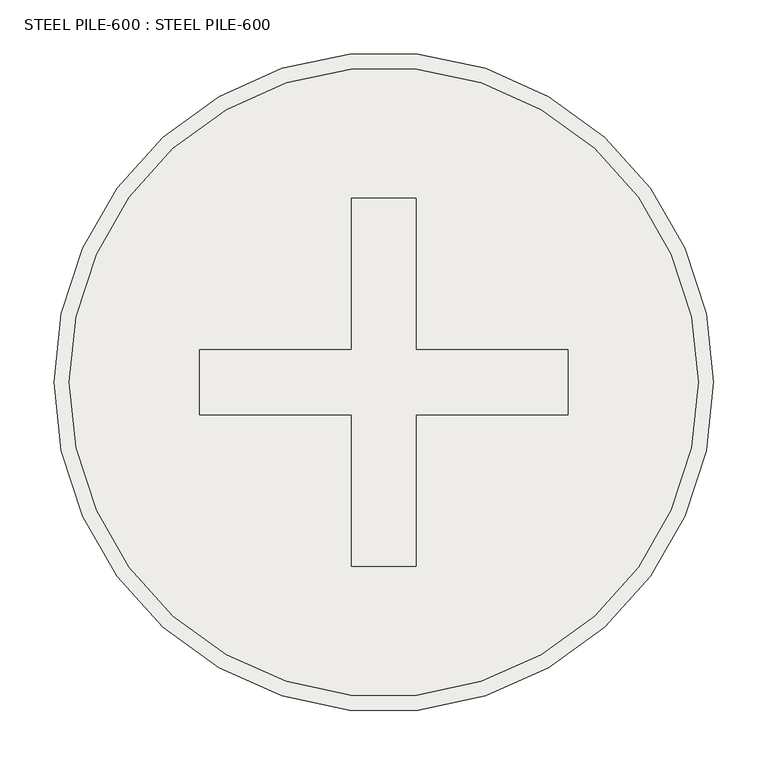
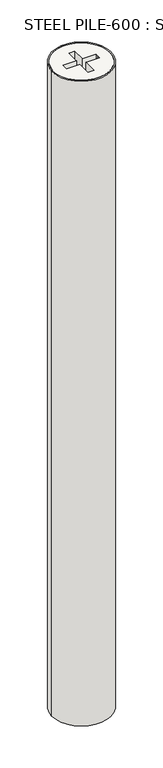
"""IFC4 building model written with IfcOpenShell, lengths in millimetres: slab geometry, STEEL PILE-600 : STEEL PILE-600."""

from ifc_helpers import new_model, si_unit, point, frame, frame_2d, origin, place, context, project, spatial, circle_curve, trimmed, segment, composite_curve, outline, extrude, source, transform, mapped, element, save
from ifc_brep_helpers import plane_surface, cylinder_surface, advanced_brep


def steel_pile_600_steel_pile_600_e2eeaf4c(model_context):
    return source(origin(), model_context, "Body", "SolidModel", [
        advanced_brep(
        [(-290.5, 19499.5208589, 150.0), (290.5, 19499.5208589, 150.0), (-30.0, 19469.5208589, 150.0), (-170.0, 19469.5208589, 150.0), (-170.0, 19499.5208589, 150.0), (-170.0, 19529.5208589, 150.0), (-30.0, 19529.5208589, 150.0), (-30.0, 19669.5208589, 150.0), (30.0, 19669.5208589, 150.0), (30.0, 19529.5208589, 150.0), (170.0, 19529.5208589, 150.0), (170.0, 19499.5208589, 150.0), (170.0, 19469.5208589, 150.0), (30.0, 19469.5208589, 150.0), (30.0, 19329.5208589, 150.0), (-30.0, 19329.5208589, 150.0), (-290.5, 19499.5208589, -1850.0), (290.5, 19499.5208589, -1850.0), (-170.0, 19469.5208589, -160.0), (-30.0, 19469.5208589, -160.0), (-30.0, 19329.5208589, -160.0), (30.0, 19329.5208589, -160.0), (30.0, 19469.5208589, -160.0), (170.0, 19469.5208589, -160.0), (170.0, 19499.5208589, -160.0), (170.0, 19529.5208589, -160.0), (30.0, 19529.5208589, -160.0), (30.0, 19669.5208589, -160.0), (-30.0, 19669.5208589, -160.0), (-30.0, 19529.5208589, -160.0), (-170.0, 19529.5208589, -160.0), (-170.0, 19499.5208589, -160.0)],
        [
            (0, 1, circle_curve(frame((0.0, 19499.5208589, 150.0), z_axis=(0.0, 0.0, 1.0), x_axis=(1.0, 0.0, 0.0)), 290.5)),
            (1, 0, circle_curve(frame((0.0, 19499.5208589, 150.0), z_axis=(0.0, 0.0, 1.0), x_axis=(1.0, 0.0, 0.0)), 290.5)),
            (2, 3),
            (3, 4),
            (4, 5),
            (5, 6),
            (6, 7),
            (7, 8),
            (8, 9),
            (9, 10),
            (10, 11),
            (11, 12),
            (12, 13),
            (13, 14),
            (14, 15),
            (15, 2),
            (16, 17, circle_curve(frame((0.0, 19499.5208589, -1850.0), z_axis=(0.0, 0.0, -1.0), x_axis=(1.0, 0.0, 0.0)), 290.5)),
            (17, 16, circle_curve(frame((0.0, 19499.5208589, -1850.0), z_axis=(0.0, 0.0, -1.0), x_axis=(1.0, 0.0, 0.0)), 290.5)),
            (0, 16),
            (17, 1),
            (18, 19),
            (19, 20),
            (20, 21),
            (21, 22),
            (22, 23),
            (23, 24),
            (24, 25),
            (25, 26),
            (26, 27),
            (27, 28),
            (28, 29),
            (29, 30),
            (30, 31),
            (31, 18),
            (18, 3),
            (2, 19),
            (15, 20),
            (14, 21),
            (13, 22),
            (12, 23),
            (11, 24),
            (10, 25),
            (9, 26),
            (8, 27),
            (7, 28),
            (6, 29),
            (5, 30),
            (4, 31),
        ],
        [
            plane_surface(frame((290.5, 19499.5208589, 150.0), z_axis=(0.0, 0.0, 1.0), x_axis=(0.0, 1.0, 0.0))),
            plane_surface(frame((290.5, 19499.5208589, -1850.0), z_axis=(0.0, 0.0, -1.0), x_axis=(0.0, -1.0, 0.0))),
            cylinder_surface(frame((0.0, 19499.5208589, -1850.0), z_axis=(0.0, 0.0, 1.0), x_axis=(1.0, 0.0, 0.0)), 290.5),
            plane_surface(frame((-170.0, 19469.5208589, -160.0), z_axis=(0.0, 0.0, 1.0), x_axis=(-1.0, 0.0, 0.0))),
            plane_surface(frame((-170.0, 19469.5208589, 160.0), z_axis=(0.0, 1.0, 0.0), x_axis=(0.0, 0.0, -1.0))),
            plane_surface(frame((-30.0, 19469.5208589, 160.0), z_axis=(1.0, 0.0, 0.0), x_axis=(0.0, 0.0, -1.0))),
            plane_surface(frame((-30.0, 19329.5208589, 160.0), z_axis=(0.0, 1.0, 0.0), x_axis=(0.0, 0.0, -1.0))),
            plane_surface(frame((30.0, 19329.5208589, 160.0), z_axis=(-1.0, 0.0, 0.0), x_axis=(0.0, 0.0, -1.0))),
            plane_surface(frame((30.0, 19469.5208589, 160.0), z_axis=(0.0, 1.0, 0.0), x_axis=(0.0, 0.0, -1.0))),
            plane_surface(frame((170.0, 19469.5208589, 160.0), z_axis=(-1.0, 0.0, 0.0), x_axis=(0.0, 0.0, -1.0))),
            plane_surface(frame((170.0, 19499.5208589, 160.0), z_axis=(-1.0, 0.0, 0.0), x_axis=(0.0, 0.0, -1.0))),
            plane_surface(frame((170.0, 19529.5208589, 160.0), z_axis=(0.0, -1.0, 0.0), x_axis=(0.0, 0.0, -1.0))),
            plane_surface(frame((30.0, 19529.5208589, 160.0), z_axis=(-1.0, 0.0, 0.0), x_axis=(0.0, 0.0, -1.0))),
            plane_surface(frame((30.0, 19669.5208589, 160.0), z_axis=(0.0, -1.0, 0.0), x_axis=(0.0, 0.0, -1.0))),
            plane_surface(frame((-30.0, 19669.5208589, 160.0), z_axis=(1.0, 0.0, 0.0), x_axis=(0.0, 0.0, -1.0))),
            plane_surface(frame((-30.0, 19529.5208589, 160.0), z_axis=(0.0, -1.0, 0.0), x_axis=(0.0, 0.0, -1.0))),
            plane_surface(frame((-170.0, 19529.5208589, 160.0), z_axis=(1.0, 0.0, 0.0), x_axis=(0.0, 0.0, -1.0))),
            plane_surface(frame((-170.0, 19499.5208589, 160.0), z_axis=(1.0, 0.0, 0.0), x_axis=(0.0, 0.0, -1.0))),
        ],
        [
            (0, [[1, 2], [3, 4, 5, 6, 7, 8, 9, 10, 11, 12, 13, 14, 15, 16]]),
            (1, [[17, 18]]),
            (2, [[-1, 19, -18, 20]]),
            (2, [[-2, -20, -17, -19]]),
            (3, [[21, 22, 23, 24, 25, 26, 27, 28, 29, 30, 31, 32, 33, 34]]),
            (4, [[-21, 35, -3, 36]]),
            (5, [[-22, -36, -16, 37]]),
            (6, [[-23, -37, -15, 38]]),
            (7, [[-24, -38, -14, 39]]),
            (8, [[-25, -39, -13, 40]]),
            (9, [[-26, -40, -12, 41]]),
            (10, [[-27, -41, -11, 42]]),
            (11, [[-28, -42, -10, 43]]),
            (12, [[-29, -43, -9, 44]]),
            (13, [[-30, -44, -8, 45]]),
            (14, [[-31, -45, -7, 46]]),
            (15, [[-32, -46, -6, 47]]),
            (16, [[-33, -47, -5, 48]]),
            (17, [[-34, -48, -4, -35]]),
        ],
    ),
        extrude(outline(composite_curve([segment(trimmed(circle_curve(frame_2d((0.0, 19499.5208589)), 304.5), [point((-304.5, 19499.5208589))], [point((304.5, 19499.5208589))], False, "CARTESIAN"), True, "CONTINUOUS"), segment(trimmed(circle_curve(frame_2d((0.0, 19499.5208589)), 304.5), [point((304.5, 19499.5208589))], [point((-304.5, 19499.5208589))], False, "CARTESIAN"), True, "CONTINUOUS")], self_intersect=False), holes=[composite_curve([segment(trimmed(circle_curve(frame_2d((0.0, 19499.5208589)), 290.5), [point((-290.5, 19499.5208589))], [point((290.5, 19499.5208589))], True, "CARTESIAN"), True, "CONTINUOUS"), segment(trimmed(circle_curve(frame_2d((0.0, 19499.5208589)), 290.5), [point((290.5, 19499.5208589))], [point((-290.5, 19499.5208589))], True, "CARTESIAN"), True, "CONTINUOUS")], self_intersect=False)]), frame((0.0, 0.0, -6850.0), z_axis=(0.0, 0.0, 1.0), x_axis=(1.0, 0.0, 0.0)), (0.0, 0.0, 1.0), 7000.0),
    ])


if __name__ == "__main__":
    model = new_model("IFC4")
    model_context = context("Model", 3, world=origin())
    ifc_project = project(units=[si_unit("LENGTHUNIT", "METRE", prefix="MILLI")], contexts=[model_context])
    site = spatial("IfcSite", under=ifc_project)
    building = spatial("IfcBuilding", under=site)
    placement = place(None, origin())
    steel_pile_600_steel_pile_600_shape = steel_pile_600_steel_pile_600_e2eeaf4c(model_context)
    element("IfcSlab", 1, ObjectType="STEEL PILE-600 : STEEL PILE-600", at=placement, inside=building, context=model_context, shape_type="MappedRepresentation", body=[
        mapped(steel_pile_600_steel_pile_600_shape, transform((0.0, 0.0, 0.0), x_axis=(1.0, 0.0, 0.0), y_axis=(0.0, 1.0, 0.0), z_axis=(0.0, 0.0, 1.0))),
    ])
    save(model, "model.ifc")
